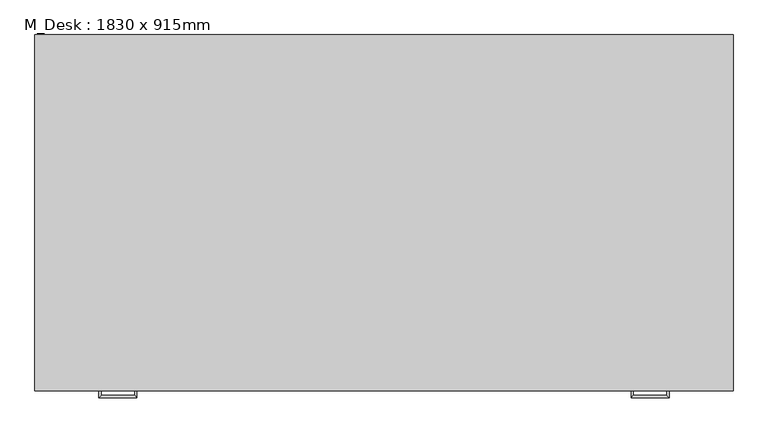
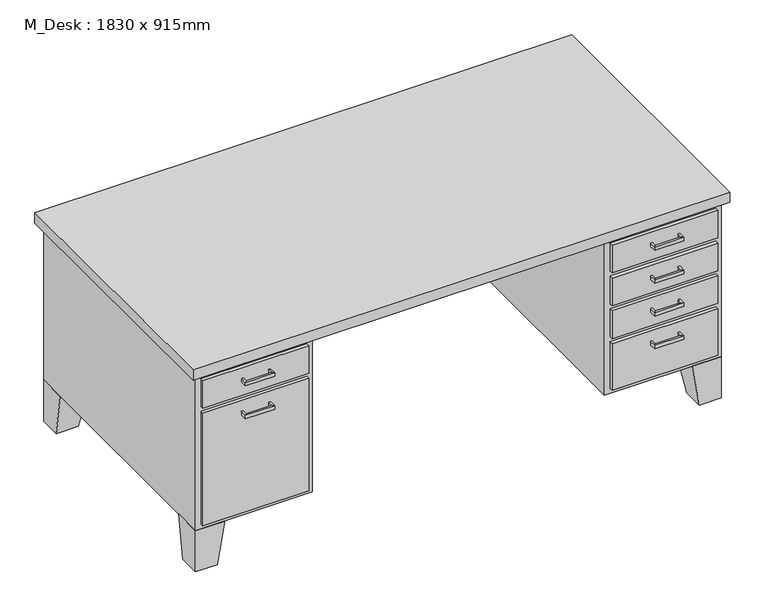
"""IFC4 building model written with IfcOpenShell, lengths in millimetres: furniture geometry, M_Desk : 1830 x 915mm."""

from ifc_helpers import new_model, si_unit, frame, origin, place, context, project, spatial, polyline, outline, extrude, faceted_brep, source, transform, mapped, element, save


def m_desk_1830_x_915mm_c290bd29(model_context):
    return source(origin(), model_context, "Body", "SolidModel", [
        extrude(outline(polyline([(-133.95, -76.5), (234.35, -76.5), (234.35, -89.2), (-133.95, -89.2), (-133.95, -76.5)])), frame((0.0, 0.0, 603.25), z_axis=(0.0, 0.0, 1.0), x_axis=(1.0, 0.0, 0.0)), (0.0, 0.0, 1.0), 101.6),
        extrude(outline(polyline([(-133.95, -76.5), (234.35, -76.5), (234.35, -89.2), (-133.95, -89.2), (-133.95, -76.5)])), frame((0.0, 0.0, 171.05), z_axis=(0.0, 0.0, 1.0), x_axis=(1.0, 0.0, 0.0)), (0.0, 0.0, 1.0), 413.15),
        extrude(outline(polyline([(1289.65, -76.5), (1657.95, -76.5), (1657.95, -89.2), (1289.65, -89.2), (1289.65, -76.5)])), frame((0.0, 0.0, 602.85), z_axis=(0.0, 0.0, 1.0), x_axis=(1.0, 0.0, 0.0)), (0.0, 0.0, 1.0), 102.0),
        extrude(outline(polyline([(1289.65, -76.5), (1657.95, -76.5), (1657.95, -89.2), (1289.65, -89.2), (1289.65, -76.5)])), frame((0.0, 0.0, 171.05), z_axis=(0.0, 0.0, 1.0), x_axis=(1.0, 0.0, 0.0)), (0.0, 0.0, 1.0), 171.45),
        extrude(outline(polyline([(1289.65, -76.5), (1657.95, -76.5), (1657.95, -89.2), (1289.65, -89.2), (1289.65, -76.5)])), frame((0.0, 0.0, 482.2), z_axis=(0.0, 0.0, 1.0), x_axis=(1.0, 0.0, 0.0)), (0.0, 0.0, 1.0), 101.6),
        extrude(outline(polyline([(1289.65, -76.5), (1657.95, -76.5), (1657.95, -89.2), (1289.65, -89.2), (1289.65, -76.5)])), frame((0.0, 0.0, 361.55), z_axis=(0.0, 0.0, 1.0), x_axis=(1.0, 0.0, 0.0)), (0.0, 0.0, 1.0), 101.6),
        faceted_brep([(-51.4, -76.5, 152.0), (-51.4, 25.1, 152.0), (-153.0, 25.1, 152.0), (-153.0, -76.5, 152.0), (-76.8, -76.5, 0.0), (-153.0, -76.5, 0.0), (-153.0, -0.3, 0.0), (-76.8, -0.3, 0.0)], [[[0, 1, 2, 3]], [[4, 5, 6, 7]], [[4, 7, 1, 0]], [[7, 6, 2, 1]], [[6, 5, 3, 2]], [[5, 4, 0, 3]]]),
        faceted_brep([(-51.4, 838.5, 152.0), (-153.0, 838.5, 152.0), (-153.0, 736.9, 152.0), (-51.4, 736.9, 152.0), (-76.8, 838.5, 0.0), (-76.8, 762.3, 0.0), (-153.0, 762.3, 0.0), (-153.0, 838.5, 0.0)], [[[0, 1, 2, 3]], [[4, 5, 6, 7]], [[4, 7, 1, 0]], [[7, 6, 2, 1]], [[6, 5, 3, 2]], [[5, 4, 0, 3]]]),
        faceted_brep([(1575.4, 838.5, 152.0), (1575.4, 736.9, 152.0), (1677.0, 736.9, 152.0), (1677.0, 838.5, 152.0), (1600.8, 838.5, 0.0), (1677.0, 838.5, 0.0), (1677.0, 762.3, 0.0), (1600.8, 762.3, 0.0)], [[[0, 1, 2, 3]], [[4, 5, 6, 7]], [[4, 7, 1, 0]], [[7, 6, 2, 1]], [[6, 5, 3, 2]], [[5, 4, 0, 3]]]),
        faceted_brep([(1575.4, -76.5, 152.0), (1677.0, -76.5, 152.0), (1677.0, 25.1, 152.0), (1575.4, 25.1, 152.0), (1600.8, -76.5, 0.0), (1600.8, -0.3, 0.0), (1677.0, -0.3, 0.0), (1677.0, -76.5, 0.0)], [[[0, 1, 2, 3]], [[4, 5, 6, 7]], [[4, 7, 1, 0]], [[7, 6, 2, 1]], [[6, 5, 3, 2]], [[5, 4, 0, 3]]]),
        extrude(outline(polyline([(-172.05, -95.55), (-172.05, 857.55), (1696.05, 857.55), (1696.05, -95.55), (-172.05, -95.55)])), frame((0.0, 0.0, 723.9), z_axis=(0.0, 0.0, 1.0), x_axis=(1.0, 0.0, 0.0)), (0.0, 0.0, 1.0), 38.1),
        extrude(outline(polyline([(1270.6, -76.5), (1270.6, 711.5), (253.4, 711.5), (253.4, -76.5), (-153.0, -76.5), (-153.0, 838.5), (1677.0, 838.5), (1677.0, -76.5), (1270.6, -76.5)])), frame((0.0, 0.0, 152.0), z_axis=(0.0, 0.0, 1.0), x_axis=(1.0, 0.0, 0.0)), (0.0, 0.0, 1.0), 571.9),
        faceted_brep([(5.75, -89.2, 546.1), (5.75, -89.2, 533.4), (-0.6, -89.2, 533.4), (-0.6, -89.2, 546.1), (5.75, -108.25, 546.1), (5.75, -108.25, 533.4), (-0.6, -114.6, 533.4), (-0.6, -114.6, 546.1), (94.65, -108.25, 546.1), (94.65, -108.25, 533.4), (101.0, -114.6, 533.4), (101.0, -114.6, 546.1), (94.65, -89.2, 546.1), (101.0, -89.2, 546.1), (101.0, -89.2, 533.4), (94.65, -89.2, 533.4)], [[[0, 1, 2, 3]], [[1, 0, 4, 5]], [[2, 1, 5, 6]], [[3, 2, 6, 7]], [[0, 3, 7, 4]], [[5, 4, 8, 9]], [[6, 5, 9, 10]], [[7, 6, 10, 11]], [[4, 7, 11, 8]], [[12, 13, 14, 15]], [[9, 8, 12, 15]], [[10, 9, 15, 14]], [[11, 10, 14, 13]], [[8, 11, 13, 12]]]),
        faceted_brep([(5.75, -89.2, 666.75), (5.75, -89.2, 654.05), (-0.6, -89.2, 654.05), (-0.6, -89.2, 666.75), (5.75, -108.25, 666.75), (5.75, -108.25, 654.05), (-0.6, -114.6, 654.05), (-0.6, -114.6, 666.75), (94.65, -108.25, 666.75), (94.65, -108.25, 654.05), (101.0, -114.6, 654.05), (101.0, -114.6, 666.75), (94.65, -89.2, 666.75), (101.0, -89.2, 666.75), (101.0, -89.2, 654.05), (94.65, -89.2, 654.05)], [[[0, 1, 2, 3]], [[1, 0, 4, 5]], [[2, 1, 5, 6]], [[3, 2, 6, 7]], [[0, 3, 7, 4]], [[5, 4, 8, 9]], [[6, 5, 9, 10]], [[7, 6, 10, 11]], [[4, 7, 11, 8]], [[12, 13, 14, 15]], [[9, 8, 12, 15]], [[10, 9, 15, 14]], [[11, 10, 14, 13]], [[8, 11, 13, 12]]]),
        faceted_brep([(1518.25, -89.2, 304.8), (1524.6, -89.2, 304.8), (1524.6, -89.2, 292.1), (1518.25, -89.2, 292.1), (1518.25, -108.25, 304.8), (1524.6, -114.6, 304.8), (1524.6, -114.6, 292.1), (1518.25, -108.25, 292.1), (1429.35, -108.25, 304.8), (1423.0, -114.6, 304.8), (1423.0, -114.6, 292.1), (1429.35, -108.25, 292.1), (1429.35, -89.2, 304.8), (1429.35, -89.2, 292.1), (1423.0, -89.2, 292.1), (1423.0, -89.2, 304.8)], [[[0, 1, 2, 3]], [[1, 0, 4, 5]], [[2, 1, 5, 6]], [[3, 2, 6, 7]], [[0, 3, 7, 4]], [[5, 4, 8, 9]], [[6, 5, 9, 10]], [[7, 6, 10, 11]], [[4, 7, 11, 8]], [[12, 13, 14, 15]], [[9, 8, 12, 15]], [[10, 9, 15, 14]], [[11, 10, 14, 13]], [[8, 11, 13, 12]]]),
        faceted_brep([(1518.25, -89.2, 425.45), (1524.6, -89.2, 425.45), (1524.6, -89.2, 412.75), (1518.25, -89.2, 412.75), (1518.25, -108.25, 425.45), (1524.6, -114.6, 425.45), (1524.6, -114.6, 412.75), (1518.25, -108.25, 412.75), (1429.35, -108.25, 425.45), (1423.0, -114.6, 425.45), (1423.0, -114.6, 412.75), (1429.35, -108.25, 412.75), (1429.35, -89.2, 425.45), (1429.35, -89.2, 412.75), (1423.0, -89.2, 412.75), (1423.0, -89.2, 425.45)], [[[0, 1, 2, 3]], [[1, 0, 4, 5]], [[2, 1, 5, 6]], [[3, 2, 6, 7]], [[0, 3, 7, 4]], [[5, 4, 8, 9]], [[6, 5, 9, 10]], [[7, 6, 10, 11]], [[4, 7, 11, 8]], [[12, 13, 14, 15]], [[9, 8, 12, 15]], [[10, 9, 15, 14]], [[11, 10, 14, 13]], [[8, 11, 13, 12]]]),
        faceted_brep([(1518.25, -89.2, 546.1), (1524.6, -89.2, 546.1), (1524.6, -89.2, 533.4), (1518.25, -89.2, 533.4), (1518.25, -108.25, 546.1), (1524.6, -114.6, 546.1), (1524.6, -114.6, 533.4), (1518.25, -108.25, 533.4), (1429.35, -108.25, 546.1), (1423.0, -114.6, 546.1), (1423.0, -114.6, 533.4), (1429.35, -108.25, 533.4), (1429.35, -89.2, 546.1), (1429.35, -89.2, 533.4), (1423.0, -89.2, 533.4), (1423.0, -89.2, 546.1)], [[[0, 1, 2, 3]], [[1, 0, 4, 5]], [[2, 1, 5, 6]], [[3, 2, 6, 7]], [[0, 3, 7, 4]], [[5, 4, 8, 9]], [[6, 5, 9, 10]], [[7, 6, 10, 11]], [[4, 7, 11, 8]], [[12, 13, 14, 15]], [[9, 8, 12, 15]], [[10, 9, 15, 14]], [[11, 10, 14, 13]], [[8, 11, 13, 12]]]),
        faceted_brep([(1518.25, -89.2, 666.75), (1524.6, -89.2, 666.75), (1524.6, -89.2, 654.05), (1518.25, -89.2, 654.05), (1518.25, -108.25, 666.75), (1524.6, -114.6, 666.75), (1524.6, -114.6, 654.05), (1518.25, -108.25, 654.05), (1429.35, -108.25, 666.75), (1423.0, -114.6, 666.75), (1423.0, -114.6, 654.05), (1429.35, -108.25, 654.05), (1429.35, -89.2, 666.75), (1429.35, -89.2, 654.05), (1423.0, -89.2, 654.05), (1423.0, -89.2, 666.75)], [[[0, 1, 2, 3]], [[1, 0, 4, 5]], [[2, 1, 5, 6]], [[3, 2, 6, 7]], [[0, 3, 7, 4]], [[5, 4, 8, 9]], [[6, 5, 9, 10]], [[7, 6, 10, 11]], [[4, 7, 11, 8]], [[12, 13, 14, 15]], [[9, 8, 12, 15]], [[10, 9, 15, 14]], [[11, 10, 14, 13]], [[8, 11, 13, 12]]]),
    ])


if __name__ == "__main__":
    model = new_model("IFC4")
    model_context = context("Model", 3, world=origin())
    ifc_project = project(units=[si_unit("LENGTHUNIT", "METRE", prefix="MILLI")], contexts=[model_context])
    site = spatial("IfcSite", under=ifc_project)
    building = spatial("IfcBuilding", under=site)
    placement = place(None, origin())
    m_desk_1830_x_915mm_shape = m_desk_1830_x_915mm_c290bd29(model_context)
    element("IfcFurniture", 1, ObjectType="M_Desk : 1830 x 915mm", at=placement, inside=building, context=model_context, shape_type="MappedRepresentation", body=[
        mapped(m_desk_1830_x_915mm_shape, transform((0.0, 0.0, 0.0), x_axis=(1.0, 0.0, 0.0), y_axis=(0.0, 1.0, 0.0), z_axis=(0.0, 0.0, 1.0))),
    ])
    save(model, "model.ifc")

# Revit data of these elements
# Type "M_Desk : 1830 x 915mm"
#   Depth = 0.915 m
#   Height = 0.762 m
#   Leg Height = 0.152 m
#   Width = 1.83 m
#   Body Material = Laminate, Ivory, Matte
#   Handle/Leg Material = Steel, Chrome Plated
#   Top Material = Cherry
#   Assembly Code = ""
# Element 1 (IfcFurniture, "M_Desk : 1830 x 915mm")
#   Materials on its faces: "Steel, Chrome Plated", "Laminate, Ivory, Matte", "Cherry"
# Materials
#   "Laminate, Ivory, Matte": class "Plastic", colour RGB 247 247 229, transparency 0, Description = "Plastic Laminate - Ivory, Matte", Cost = 0
#   "Steel, Chrome Plated": class "Metal", colour RGB 244 244 244, transparency 0, Description = "Chromiuim plated steel", Cost = 0
#   "Cherry": class "Wood", colour RGB 154 107 61, transparency 0, Description = "Prunus Serotina", Cost = 0
